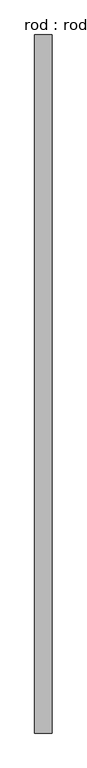
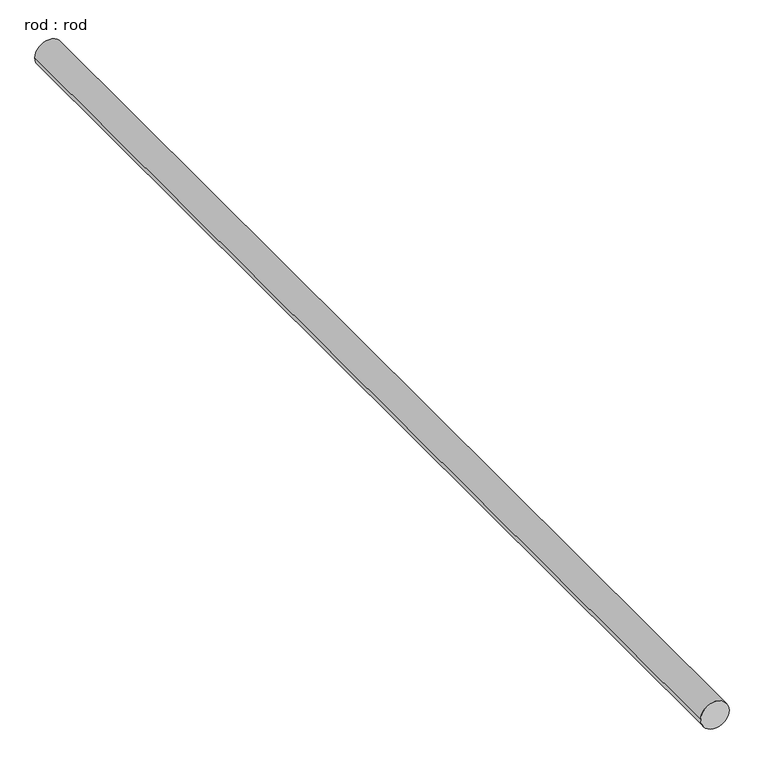
"""IFC4 building model written with IfcOpenShell, lengths in millimetres: proxy geometry, rod : rod."""

from ifc_helpers import new_model, si_unit, point, frame, frame_2d, origin, place, context, project, spatial, circle_curve, trimmed, segment, composite_curve, outline, extrude, source, transform, mapped, element, save


def rod_rod_94924a5e(model_context):
    return source(origin(), model_context, "Body", "SweptSolid", [
        extrude(outline(composite_curve([segment(trimmed(circle_curve(frame_2d((0.0108462, 0.0)), 200.0), [point((0.0108462, 200.0))], [point((0.0108462, -200.0))], False, "CARTESIAN"), True, "CONTINUOUS"), segment(trimmed(circle_curve(frame_2d((0.0108462, 0.0)), 200.0), [point((0.0108462, -200.0))], [point((0.0108462, 200.0))], False, "CARTESIAN"), True, "CONTINUOUS")], self_intersect=False)), frame((0.0, -4022.7121035, 0.0), z_axis=(0.0, 1.0, 0.0), x_axis=(0.0, 0.0, 1.0)), (0.0, 0.0, 1.0), 16230.8814377),
    ])


if __name__ == "__main__":
    model = new_model("IFC4")
    model_context = context("Model", 3, world=origin())
    ifc_project = project(units=[si_unit("LENGTHUNIT", "METRE", prefix="MILLI")], contexts=[model_context])
    site = spatial("IfcSite", under=ifc_project)
    building = spatial("IfcBuilding", under=site)
    placement = place(None, origin())
    rod_rod_shape = rod_rod_94924a5e(model_context)
    element("IfcBuildingElementProxy", 1, Name="rod : rod", ObjectType="rod : rod", at=placement, inside=building, context=model_context, shape_type="MappedRepresentation", body=[
        mapped(rod_rod_shape, transform((0.0, 0.0, 0.0), x_axis=(1.0, 0.0, 0.0), y_axis=(0.0, 1.0, 0.0), z_axis=(0.0, 0.0, 1.0))),
    ])
    save(model, "model.ifc")

# Revit data of these elements
# Type "rod : rod"
#   Default Elevation = 0
